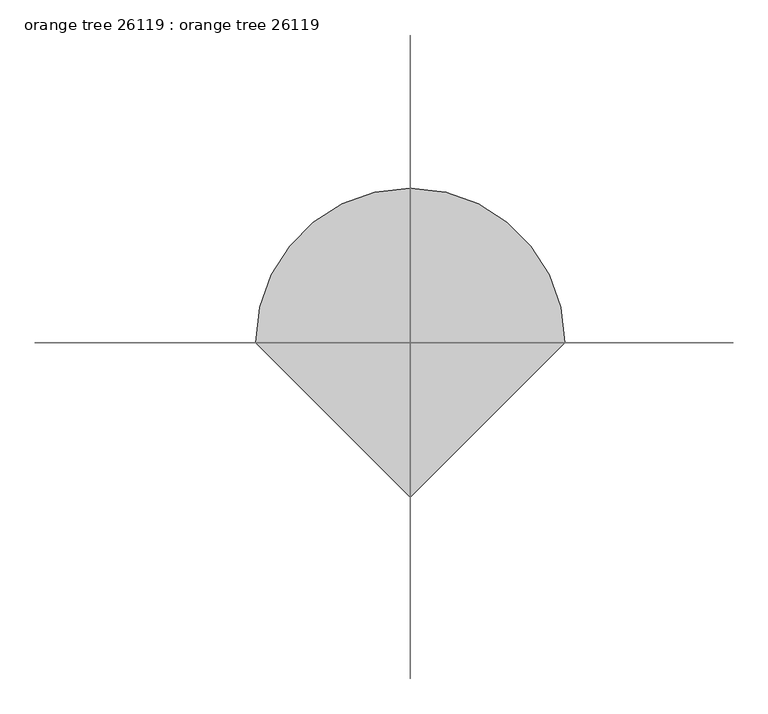
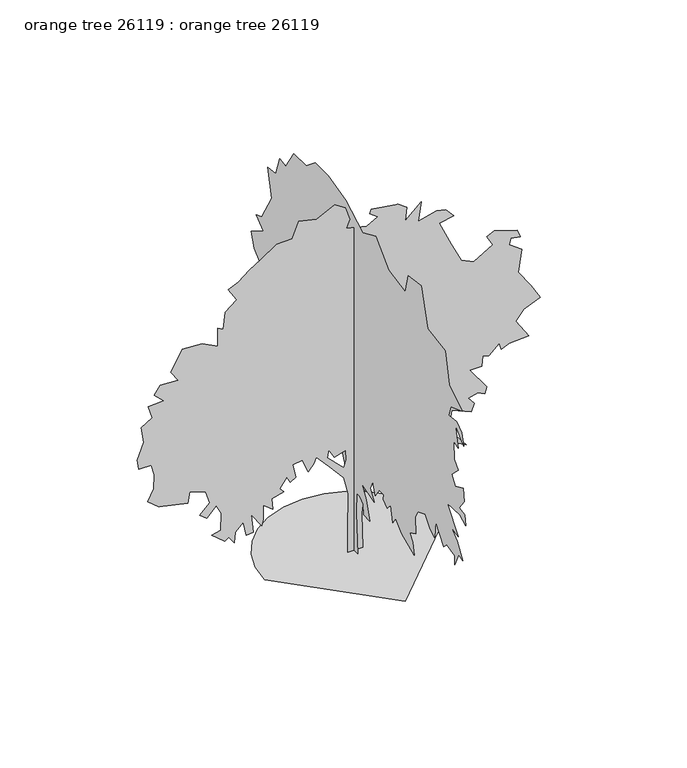
"""IFC4 building model written with IfcOpenShell, lengths in millimetres: proxy geometry, orange tree 26119 : orange tree 26119."""

from ifc_helpers import new_model, si_unit, origin, place, context, project, spatial, triangles, source, transform, mapped, element, save


def orange_tree_26119_orange_tree_26119_f1cce5cf(model_context):
    return source(origin(), model_context, "Body", "Tessellation", [
        triangles([(-803.9534712, 0.0, 6.05e-05), (-782.6987366, 184.2127929, 6.05e-05), (-722.1679836, 353.3826814, 6.05e-05), (-627.2075008, 502.663613, 6.05e-05), (-502.663613, 627.2075008, 6.05e-05), (-353.3826814, 722.1679836, 6.05e-05), (-184.2125386, 782.6987366, 6.05e-05), (3.51e-05, 803.9534712, 6.05e-05), (184.2127929, 782.6987366, 6.05e-05), (353.3826814, 722.1679836, 6.05e-05), (502.663613, 627.2075008, 6.05e-05), (627.2075008, 502.663613, 6.05e-05), (722.1679836, 353.3826814, 6.05e-05), (782.6987366, 184.2125386, 6.05e-05), (803.9534712, -7.03e-05, 6.05e-05), (-0.0001054, -803.9534712, 6.05e-05), (-4.73e-05, 77.0963933, 4.81e-05), (-2.95e-05, 72.7562921, 588.9525321), (-2.7e-05, 181.2628458, 836.3460434), (-3.2e-05, 320.1518609, 875.4087753), (-3.63e-05, 346.1919502, 771.2433311), (-3.87e-05, 472.0617019, 879.7495714), (-4.71e-05, 532.8235817, 688.7770712), (-4.92e-05, 632.6507006, 766.9024624), (-5.78e-05, 693.4151602, 571.5916368), (-5.81e-05, 775.878804, 684.4387459), (-6.3e-05, 832.3023949, 606.3134274), (-6.59e-05, 979.8713671, 727.8398031), (-5.62e-05, 875.7059229, 897.110503), (-4.32e-05, 610.9489002, 936.1731623), (-5.12e-05, 849.6633265, 1027.3185436), (-5.75e-05, 1031.9540892, 1088.0830032), (-6.35e-05, 1166.5029985, 1088.0830032), (-6.17e-05, 1201.224789, 1200.9301849), (-6.47e-05, 1296.7111118, 1244.3311695), (-5.59e-05, 1244.6283897, 1461.3462662), (-6.14e-05, 1422.5782837, 1543.8099827), (-6.28e-05, 1578.8289207, 1730.4416142), (-5.38e-05, 1452.9591328, 1843.2887959), (-5.55e-05, 1552.7863243, 1938.7749733), (-5.37e-05, 1600.5281776, 2068.9830139), (-4.21e-05, 1418.2374149, 2186.1685936), (-4.43e-05, 1526.7437279, 2272.9730335), (-3.95e-05, 1439.9391426, 2303.3564987), (-2.42e-05, 1279.3501076, 2576.8055054), (-1.94e-05, 1344.4529652, 2837.2061806), (-1.34e-05, 1218.5857206, 2850.2364899), (-5.3e-06, 1157.821261, 3028.1889999), (-1.5e-06, 1062.3375544, 3015.1586906), (9.7e-06, 940.8087078, 3206.14151), (1.89e-05, 741.1570135, 3214.8028999), (2.81e-05, 606.6080678, 3323.3116837), (3.75e-05, 398.2746723, 3327.6550232), (4.77e-05, 124.839264, 3258.2115875), (5.48e-05, -135.5766083, 3106.2941162), (6.66e-05, -339.5701524, 3197.4545403), (6.98e-05, -543.560172, 2997.8106216), (7.98e-05, -799.6379642, 2950.0585945), (8.73e-05, -847.3798176, 3128.0111046), (9.73e-05, -1051.3723806, 3158.3894829), (9.14e-05, -1151.1994995, 2811.1714325), (0.0001025, -1428.9739689, 2767.7627449), (9.64e-05, -1485.3975597, 2476.9656693), (0.0001018, -1689.3900501, 2351.0983521), (9.21e-05, -1515.7810249, 2285.9956398), (8.75e-05, -1481.0591618, 2186.1685936), (9.36e-05, -1606.926479, 2199.1910545), (9.54e-05, -1685.0517975, 2142.767609), (9.34e-05, -1715.4327919, 2029.9204273), (9.11e-05, -1580.8837372, 2155.7875992), (8.77e-05, -1632.9664593, 1964.815099), (8.51e-05, -1559.1820095, 1986.5168266), (8.02e-05, -1563.5228783, 1817.2460541), (8.14e-05, -1632.9664593, 1752.1433418), (7.34e-05, -1524.4602917, 1647.9754269), (7.38e-05, -1585.2246059, 1569.8525791), (8.13e-05, -1711.0919231, 1630.6144226), (7.79e-05, -1719.7736607, 1504.7472507), (7.16e-05, -1645.9890656, 1404.9226753), (7.48e-05, -1728.4527821, 1387.5618164), (7.27e-05, -1745.813641, 1292.0754936), (6.99e-05, -1650.3299343, 1339.817347), (6.11e-05, -1459.3574341, 1331.1382256), (6.23e-05, -1628.6282066, 1118.463925), (5.81e-05, -1520.1218937, 1140.1657253), (5.99e-05, -1611.2673477, 1062.0404068), (5.99e-05, -1698.0717876, 931.8322935), (5.77e-05, -1637.307328, 949.1932251), (5.11e-05, -1576.5454845, 818.9851845), (5.33e-05, -1572.2046158, 901.4513718), (4.88e-05, -1450.6756966, 931.8322935), (4.52e-05, -1402.9338432, 884.0904402), (4.47e-05, -1281.4075401, 1049.020344), (3.92e-05, -1264.0440651, 888.4313089), (3.71e-05, -1194.6004841, 923.1530994), (3.64e-05, -1116.4751656, 1018.6394222), (2.99e-05, -999.2896585, 975.2358215), (2.55e-05, -955.8861305, 892.7696342), (2.14e-05, -964.567868, 740.8623367), (1.6e-05, -873.4224867, 697.4588087), (1.6e-05, -916.8234713, 632.353553), (1.37e-05, -938.5251989, 523.8472401), (7.6e-06, -743.2143734, 610.6542961), (6.3e-06, -656.4073174, 697.4588087), (2.2e-06, -608.665464, 632.353553), (5.3e-06, -578.2845423, 779.9225252), (9e-07, -521.8609514, 719.1606091), (-7e-07, -456.7556594, 762.5615936), (1.1e-06, -465.4373606, 810.3059904), (-2e-06, -395.9937432, 810.3059904), (-7.3e-06, -335.22932, 723.5014778), (-6e-06, -291.8257738, 832.0077181), (-1e-05, -257.1039651, 749.5415308), (-1.02e-05, -317.8683884, 649.7169554), (-1.72e-05, -122.5560549, 710.4788715), (-1.74e-05, -192.000181, 597.6317262), (-2.03e-05, -244.0831574, 424.0226646), (-2.39e-05, -157.2781179, 432.7018224), (-2.16e-05, -144.2573102, 528.1880725), (-2.27e-05, -92.1740885, 571.5916368), (-2.48e-05, -44.4312178, 571.5916368), (-3.04e-05, -40.0908669, 389.3008378), (-4.11e-05, -61.7923765, 5.22e-05), (-2.23e-05, 137.8603261, 927.4914248), (-2.41e-05, 124.8395184, 849.3686497), (-2.39e-05, 33.6941257, 719.1606091), (-1.71e-05, 3.3121102, 901.4513718), (-1.8e-05, 64.07584, 962.2158314), (58.7260893, -2.69e-05, 920.6994701), (38.9260215, -3.03e-05, 877.8014345), (32.3258294, -4.22e-05, 683.1001648), (45.5259593, -4.5e-05, 626.9992287), (78.5256484, -3.59e-05, 755.7010386), (104.9259083, -2.72e-05, 881.1008698), (-56.7740963, -8.68e-05, 0.0), (-53.4738754, -7.45e-05, 204.6001204), (-50.1739042, -5.35e-05, 554.4008984), (-93.0740155, -4.51e-05, 726.0008165), (-225.0743068, -4.16e-05, 881.1008698), (-337.2739989, -3.93e-05, 1003.2012657), (-363.6747857, -4.36e-05, 950.3996922), (-409.8748363, -4.89e-05, 894.3012995), (-465.9733017, -4.39e-05, 1019.7011307), (-551.7745325, -4.85e-05, 1006.500701), (-522.0743105, -5.46e-05, 881.1008698), (-574.8733043, -5.89e-05, 848.1012125), (-604.5735263, -5.67e-05, 907.4991131), (-667.2734419, -6.47e-05, 818.4009905), (-634.2737846, -6.56e-05, 778.799774), (-739.8743156, -7.2e-05, 749.099552), (-729.9733938, -7.77e-05, 646.8010723), (-819.0740599, -7.74e-05, 716.0998947), (-815.7746246, -8.54e-05, 580.7991417), (-832.2744169, -8.94e-05, 524.7006763), (-924.6745909, -8.52e-05, 663.3008646), (-904.8752907, -9.48e-05, 488.3989677), (-970.8746778, -9.8e-05, 481.8000609), (-997.2754646, -9.11e-05, 617.1008503), (-1069.8737223, -9.86e-05, 544.4999765), (-1079.7746441, -0.0001046, 452.0998389), (-1129.2741663, -0.0001028, 518.0991898), (-1165.5758749, -0.0001058, 495.0004543), (-1281.0748569, -0.0001051, 590.7000635), (-1201.8750401, -0.0001005, 610.4993637), (-1195.2735535, -9.05e-05, 772.2009035), (-1241.4736404, -8.73e-05, 861.2990261), (-1327.2749439, -9.65e-05, 768.9013956), (-1389.9747505, -9.61e-05, 821.7004257), (-1300.8740845, -8.71e-05, 907.4991131), (-1337.1733223, -8.2e-05, 1019.7011307), (-1479.0755619, -8.49e-05, 1075.799596), (-1495.5752815, -9.19e-05, 970.2015358), (-1759.5754463, -9.97e-05, 1032.9014877), (-1858.5744907, -9.91e-05, 1115.4007399), (-1805.7755333, -9.07e-05, 1217.6992195), (-1799.1740467, -8.25e-05, 1349.70061), (-1825.5747608, -7.76e-05, 1451.999017), (-1937.7743076, -8.27e-05, 1448.6996544), (-1950.9746647, -7.78e-05, 1541.0998283), (-1894.8735832, -6.63e-05, 1692.9004463), (-1917.9749348, -5.84e-05, 1841.4015564), (-1815.6739117, -5.04e-05, 1900.7993843), (-1855.2749828, -4.52e-05, 2016.3009098), (-1713.3753593, -3.86e-05, 2022.8997803), (-1799.1740467, -3.75e-05, 2105.4015759), (-1746.3750893, -3.05e-05, 2184.6013927), (-1584.6734768, -2.4e-05, 2174.7003983), (-1650.6754074, -2.1e-05, 2273.6994427), (-1548.3743843, -5.5e-06, 2458.4999359), (-1366.8735443, 1.9e-06, 2448.6014122), (-1228.2732834, 3.6e-06, 2376.0006111), (-1228.2732834, 1.38e-05, 2547.5953697), (-1178.7737612, 1.44e-05, 2521.1995972), (-1158.974461, 2.45e-05, 2676.2973976), (-1056.6733652, 3.39e-05, 2758.7964317), (-1132.5736742, 3.79e-05, 2880.8942116), (-1040.1735003, 4.41e-05, 2917.1908333), (-941.1744558, 5.33e-05, 2999.6901581), (-835.5739248, 6.19e-05, 3065.7047333), (-693.6742287, 7.36e-05, 3158.1101395), (-555.0740041, 7.98e-05, 3161.4119728), (-495.6735237, 9.13e-05, 3309.9005836), (-333.9745637, 9.62e-05, 3273.6039619), (-172.2735144, 0.000108, 3352.8011627), (-79.8736311, 0.0001083, 3290.0884209), (-36.9737765, 0.0001029, 3167.990641), (-66.673751, 9.71e-05, 3092.0952736), (114.8263214, 0.0001024, 3049.1946945), (213.8264105, 0.0001101, 3105.303479), (144.5262982, 0.00011, 3154.8080154), (154.426457, 0.0001128, 3194.4067612), (401.9271747, 0.0001213, 3154.8080154), (477.8274837, 0.0001215, 3102.001355), (461.327655, 0.0001133, 2976.6014511), (606.5267864, 0.0001275, 3108.6053123), (580.126036, 0.0001159, 2933.700872), (745.1270473, 0.0001255, 2973.2996178), (827.6262268, 0.0001279, 2953.5130348), (900.2271006, 0.0001263, 2874.2902542), (768.2257828, 0.000119, 2847.8997139), (877.125749, 0.0001096, 2610.3081116), (929.9273226, 0.0001052, 2498.1010071), (969.525923, 0.0001024, 2422.2006981), (1078.4258892, 0.0001042, 2372.7011032), (1253.3278587, 0.000118, 2474.9995102), (1197.2268499, 0.0001212, 2570.7093658), (1266.525745, 0.000126, 2600.4020302), (1474.4272991, 0.0001312, 2534.4002449), (1497.5260345, 0.0001279, 2461.8017693), (1415.0268551, 0.0001252, 2478.3016342), (1401.826498, 0.0001211, 2418.9011902), (1514.0258995, 0.0001213, 2339.7013733), (1481.0261696, 0.0001075, 2131.7998192), (1593.2257164, 0.0001027, 1970.1008228), (1679.0268745, 9.78e-05, 1824.9016914), (1530.5257645, 8.76e-05, 1762.1992687), (1457.9274342, 7.91e-05, 1673.1010735), (1576.7258514, 7.35e-05, 1491.6002335), (1398.5269901, 6.51e-05, 1481.6993843), (1329.2255516, 6.03e-05, 1451.999017), (1309.4263241, 6.32e-05, 1514.701585), (1213.7267149, 5.39e-05, 1428.9002815), (1160.9276848, 5.24e-05, 1442.1006386), (1151.026763, 4.66e-05, 1352.9999725), (1045.426232, 4.18e-05, 1349.70061), (1197.2268499, 3.59e-05, 1138.4994753), (1180.726985, 3.16e-05, 1079.1015747), (1114.7275978, 3.05e-05, 1108.7992533), (1032.2258749, 2.57e-05, 1088.9999531), (1085.0273758, 2.39e-05, 1019.7011307), (1058.626589, 1.86e-05, 950.3996922), (883.7272356, 1.53e-05, 1023.0005659), (854.0270136, 3.8e-06, 851.4006477), (1012.4265747, -1.3e-06, 650.1005075), (877.125749, -2.7e-06, 726.0008165), (830.9257347, -1.63e-05, 531.2995831), (801.2255127, -1.04e-05, 653.3999428), (745.1270473, -8.7e-06, 722.7013813), (642.8259516, -1.59e-05, 676.5012943), (586.7274862, -2.47e-05, 570.900727), (487.725862, -2.15e-05, 696.3005945), (392.0262528, -1.76e-05, 831.6013475), (349.1256374, -2.48e-05, 742.5006815), (316.1259439, -1.76e-05, 887.6998129), (187.4264049, -2.7e-05, 824.999861), (114.8263214, -3.72e-05, 706.1989729), (71.9262193, -6.15e-05, 329.999443), (81.8261282, -8.08e-05, 0.0001067), (-178.8742198, -3.57e-05, 947.1002569), (-228.3742689, -3.25e-05, 1036.200923), (-238.2741733, -3.73e-05, 963.6001219), (-89.7740443, -3.95e-05, 818.4009905), (-66.6740053, -3.43e-05, 887.6998129), (-73.2739431, -2.91e-05, 980.0999868)], [[16, 15, 1], [15, 14, 1], [1, 14, 2], [14, 13, 2], [2, 13, 3], [3, 13, 4], [13, 12, 4], [12, 11, 4], [4, 11, 5], [5, 11, 6], [6, 11, 7], [7, 11, 8], [8, 11, 9], [9, 11, 10], [17, 126, 18], [89, 88, 90], [69, 68, 70], [68, 67, 70], [84, 83, 85], [87, 86, 88], [18, 126, 19], [126, 125, 19], [114, 113, 115], [105, 104, 106], [64, 63, 65], [81, 80, 82], [80, 79, 82], [67, 66, 70], [25, 24, 26], [102, 101, 103], [111, 110, 112], [43, 42, 44], [71, 70, 72], [21, 20, 22], [101, 100, 103], [117, 116, 118], [118, 116, 119], [77, 76, 78], [23, 22, 24], [94, 93, 95], [95, 93, 96], [78, 76, 79], [92, 91, 93], [46, 45, 47], [119, 116, 120], [116, 115, 120], [27, 26, 28], [28, 26, 29], [29, 26, 30], [26, 24, 30], [24, 22, 30], [17, 123, 126], [123, 122, 126], [122, 121, 126], [74, 73, 75], [82, 79, 83], [79, 76, 83], [38, 37, 39], [125, 124, 19], [60, 59, 61], [59, 58, 61], [107, 106, 108], [108, 106, 109], [70, 66, 72], [19, 124, 20], [35, 34, 36], [48, 47, 49], [103, 100, 104], [120, 115, 121], [121, 115, 126], [126, 115, 127], [41, 40, 42], [40, 39, 42], [33, 32, 34], [115, 113, 127], [113, 112, 127], [62, 61, 63], [56, 55, 57], [99, 98, 100], [100, 98, 104], [104, 98, 106], [88, 86, 90], [90, 86, 91], [86, 85, 91], [91, 85, 93], [85, 83, 93], [76, 75, 83], [37, 36, 39], [50, 49, 51], [93, 83, 96], [34, 32, 36], [98, 97, 106], [32, 31, 36], [44, 42, 45], [106, 97, 109], [52, 51, 53], [83, 75, 96], [96, 75, 97], [63, 61, 65], [65, 61, 66], [61, 58, 66], [58, 57, 66], [97, 75, 109], [75, 73, 109], [73, 72, 109], [72, 66, 109], [66, 57, 109], [109, 57, 110], [110, 57, 112], [112, 57, 127], [127, 57, 128], [57, 55, 128], [55, 54, 128], [54, 53, 128], [53, 51, 128], [51, 49, 128], [49, 47, 128], [47, 45, 128], [45, 42, 128], [42, 39, 128], [39, 36, 128], [36, 31, 128], [31, 30, 128], [128, 30, 124], [124, 30, 20], [20, 30, 22], [130, 135, 131], [135, 130, 136], [136, 130, 137], [131, 135, 132], [254, 253, 255], [256, 255, 257], [137, 130, 138], [129, 272, 130], [130, 272, 138], [272, 129, 273], [263, 262, 264], [215, 214, 216], [138, 272, 139], [272, 271, 139], [139, 271, 140], [160, 159, 161], [151, 150, 152], [154, 153, 155], [153, 152, 155], [163, 162, 164], [219, 218, 220], [238, 237, 239], [229, 228, 230], [228, 227, 230], [192, 191, 193], [142, 141, 143], [149, 148, 150], [260, 259, 261], [183, 182, 184], [218, 217, 220], [162, 161, 164], [271, 270, 140], [273, 129, 274], [196, 195, 197], [135, 268, 132], [268, 267, 132], [267, 266, 132], [132, 266, 133], [266, 265, 133], [133, 265, 134], [247, 246, 248], [246, 245, 248], [235, 234, 236], [141, 140, 143], [226, 225, 227], [227, 225, 230], [230, 225, 231], [168, 167, 169], [167, 166, 169], [240, 239, 241], [146, 145, 147], [145, 144, 147], [257, 255, 258], [255, 253, 258], [172, 171, 173], [239, 237, 241], [217, 216, 220], [248, 245, 249], [251, 250, 252], [250, 249, 252], [156, 155, 157], [157, 155, 158], [211, 210, 212], [210, 209, 212], [178, 177, 179], [244, 243, 245], [202, 201, 203], [185, 184, 186], [186, 184, 187], [269, 274, 270], [174, 173, 175], [173, 171, 175], [161, 159, 164], [179, 177, 180], [159, 158, 164], [164, 158, 165], [158, 155, 165], [175, 171, 176], [181, 180, 182], [189, 188, 190], [188, 187, 190], [190, 187, 191], [232, 231, 233], [249, 245, 252], [213, 212, 214], [212, 209, 214], [204, 203, 205], [205, 203, 206], [206, 203, 207], [203, 201, 207], [265, 264, 134], [209, 208, 214], [242, 241, 243], [231, 225, 233], [225, 224, 233], [234, 233, 236], [233, 224, 236], [236, 224, 237], [237, 224, 241], [241, 224, 243], [224, 223, 243], [243, 223, 245], [155, 152, 165], [165, 152, 166], [261, 259, 262], [259, 258, 262], [258, 253, 262], [253, 252, 262], [262, 252, 264], [252, 245, 264], [245, 223, 264], [264, 223, 134], [134, 223, 129], [129, 223, 274], [274, 223, 270], [223, 222, 270], [222, 221, 270], [221, 220, 270], [220, 216, 270], [216, 214, 270], [214, 208, 270], [208, 207, 270], [207, 201, 270], [201, 200, 270], [200, 199, 270], [199, 198, 270], [198, 197, 270], [197, 195, 270], [195, 194, 270], [194, 193, 270], [193, 191, 270], [270, 191, 140], [140, 191, 143], [143, 191, 144], [191, 187, 144], [187, 184, 144], [184, 182, 144], [182, 180, 144], [180, 177, 144], [177, 176, 144], [176, 171, 144], [171, 170, 144], [144, 170, 147], [170, 169, 147], [169, 166, 147], [166, 152, 147], [147, 152, 148], [148, 152, 150]], closed=False),
    ])


if __name__ == "__main__":
    model = new_model("IFC4")
    model_context = context("Model", 3, world=origin())
    ifc_project = project(units=[si_unit("LENGTHUNIT", "METRE", prefix="MILLI")], contexts=[model_context])
    site = spatial("IfcSite", under=ifc_project)
    building = spatial("IfcBuilding", under=site)
    placement = place(None, origin())
    orange_tree_26119_orange_tree_26119_shape = orange_tree_26119_orange_tree_26119_f1cce5cf(model_context)
    element("IfcBuildingElementProxy", 1, Name="orange tree 26119 : orange tree 26119", ObjectType="orange tree 26119 : orange tree 26119", at=placement, inside=building, context=model_context, shape_type="MappedRepresentation", body=[
        mapped(orange_tree_26119_orange_tree_26119_shape, transform((0.0, 0.0, 0.0), x_axis=(1.0, 0.0, 0.0), y_axis=(0.0, 1.0, 0.0), z_axis=(0.0, 0.0, 1.0))),
    ])
    save(model, "model.ifc")

# Revit data of these elements
# Type "orange tree 26119 : orange tree 26119"
#   built-in parameter 1005195 = "RPC-16-FVGW-4XXX-7J75-W000-ST1L-LVER-AU"
#   Height = 0
